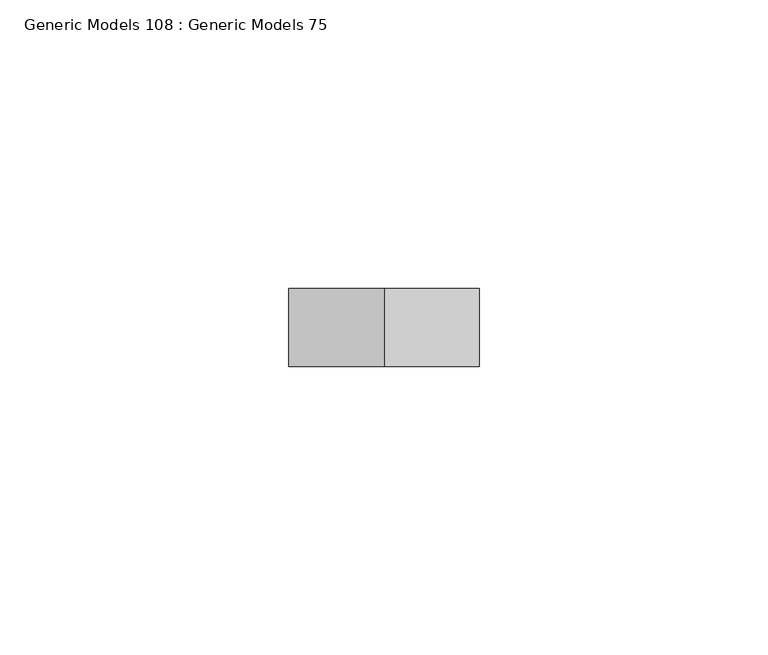
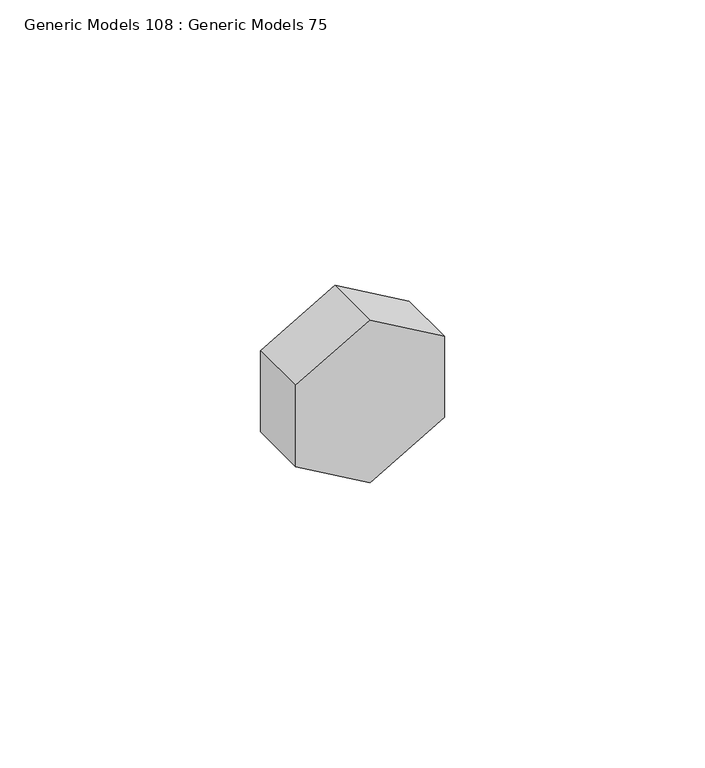
"""IFC4 building model written with IfcOpenShell, lengths in millimetres: proxy geometry, Generic Models 108 : Generic Models 75."""

from ifc_helpers import new_model, si_unit, frame, origin, place, context, project, spatial, polyline, outline, extrude, source, transform, mapped, element, save


def generic_models_108_generic_models_75_49776081(model_context):
    return source(origin(), model_context, "Body", "SweptSolid", [
        extrude(outline(polyline([(268485.9375, 31991.9073871), (268504.9875, 31991.9073871), (268514.5125, 31975.4096032), (268504.9875, 31958.9118192), (268485.9375, 31958.9118192), (268476.4125, 31975.4096032), (268485.9375, 31991.9073871)])), frame((0.0, 30858.4781612, 0.0), z_axis=(0.0, 1.0, 0.0), x_axis=(0.0, 0.0, 1.0)), (0.0, 0.0, 1.0), 13.49375),
    ])


if __name__ == "__main__":
    model = new_model("IFC4")
    model_context = context("Model", 3, world=origin())
    ifc_project = project(units=[si_unit("LENGTHUNIT", "METRE", prefix="MILLI")], contexts=[model_context])
    site = spatial("IfcSite", under=ifc_project)
    building = spatial("IfcBuilding", under=site)
    placement = place(None, origin())
    generic_models_108_generic_models_75_shape = generic_models_108_generic_models_75_49776081(model_context)
    element("IfcBuildingElementProxy", 1, Name="Generic Models 108 : Generic Models 75", ObjectType="Generic Models 108 : Generic Models 75", at=placement, inside=building, context=model_context, shape_type="MappedRepresentation", body=[
        mapped(generic_models_108_generic_models_75_shape, transform((0.0, 0.0, 0.0), x_axis=(1.0, 0.0, 0.0), y_axis=(0.0, 1.0, 0.0), z_axis=(0.0, 0.0, 1.0))),
    ])
    save(model, "model.ifc")
